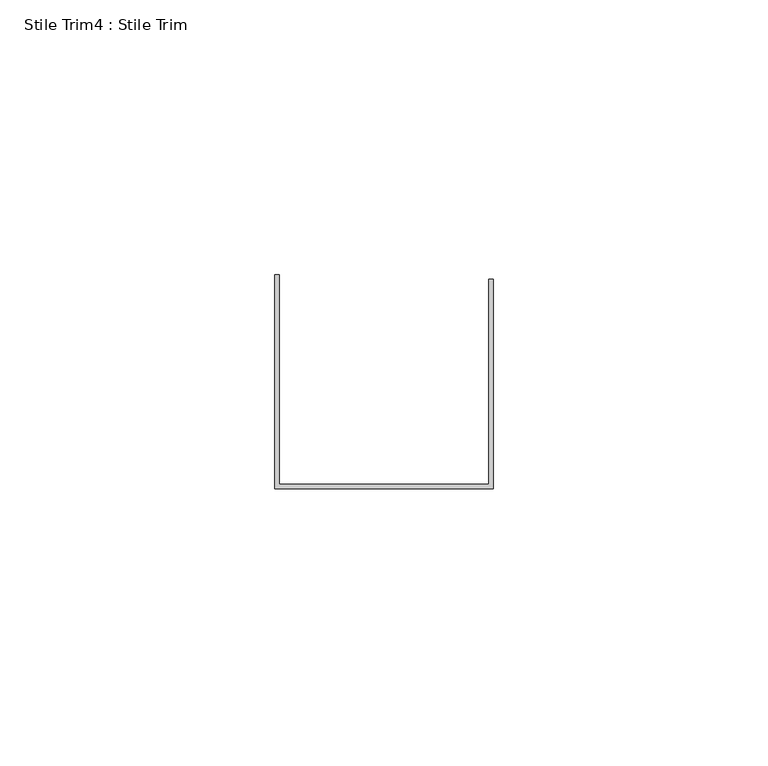
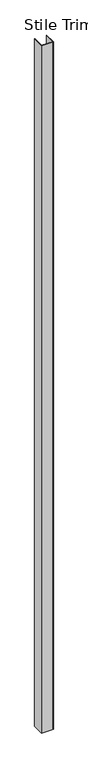
"""IFC4 building model written with IfcOpenShell, lengths in millimetres: proxy geometry, Stile Trim4 : Stile Trim."""

from ifc_helpers import new_model, si_unit, frame, origin, place, context, project, spatial, polyline, outline, extrude, source, transform, mapped, element, save


def stile_trim4_stile_trim_8294cd2f(model_context):
    return source(origin(), model_context, "Body", "SweptSolid", [
        extrude(outline(polyline([(587327.0060739, -536420.7663841), (587327.0060739, -536381.8789841), (587327.7934739, -536381.8789841), (587327.7934739, -536419.9789841), (587365.8934739, -536419.9789841), (587365.8934739, -536382.6663841), (587366.6808739, -536382.6663841), (587366.6808739, -536420.7663841), (587327.0060739, -536420.7663841)])), frame((0.0, 0.0, 12.7), z_axis=(0.0, 0.0, 1.0), x_axis=(1.0, 0.0, 0.0)), (0.0, 0.0, 1.0), 2425.7),
    ])


if __name__ == "__main__":
    model = new_model("IFC4")
    model_context = context("Model", 3, world=origin())
    ifc_project = project(units=[si_unit("LENGTHUNIT", "METRE", prefix="MILLI")], contexts=[model_context])
    site = spatial("IfcSite", under=ifc_project)
    building = spatial("IfcBuilding", under=site)
    placement = place(None, origin())
    stile_trim4_stile_trim_shape = stile_trim4_stile_trim_8294cd2f(model_context)
    element("IfcBuildingElementProxy", 1, Name="Stile Trim4 : Stile Trim", ObjectType="Stile Trim4 : Stile Trim", at=placement, inside=building, context=model_context, shape_type="MappedRepresentation", body=[
        mapped(stile_trim4_stile_trim_shape, transform((0.0, 0.0, 0.0), x_axis=(1.0, 0.0, 0.0), y_axis=(0.0, 1.0, 0.0), z_axis=(0.0, 0.0, 1.0))),
    ])
    save(model, "model.ifc")

# Revit data of these elements
# Element 1 (IfcBuildingElementProxy, "Stile Trim4 : Stile Trim")
#   Materials on its faces: "EDGE TRIM BY MTL PANEL MFR."
# Materials
#   "EDGE TRIM BY MTL PANEL MFR.": class "Generic", colour RGB 239 242 240, transparency 0, Cost = 0
